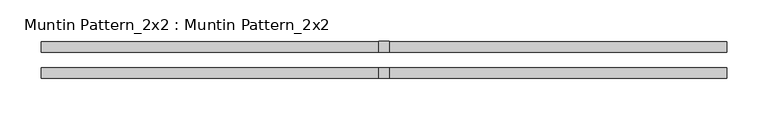
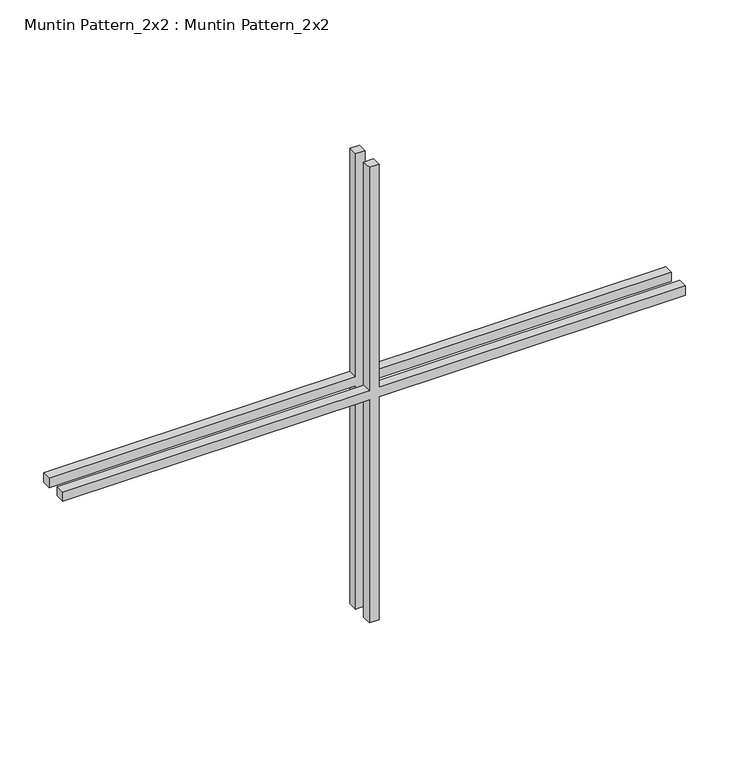
"""IFC4 building model written with IfcOpenShell, lengths in millimetres: proxy geometry, Muntin Pattern_2x2 : Muntin Pattern_2x2."""

from ifc_helpers import new_model, si_unit, frame, origin, place, context, project, spatial, polyline, outline, extrude, source, transform, mapped, element, save


def muntin_pattern_2x2_muntin_pattern_2x2_6dda0405(model_context):
    return source(origin(), model_context, "Body", "SweptSolid", [
        extrude(outline(polyline([(325.4375, -6.35), (325.4375, -412.75), (312.7375, -412.75), (312.7375, -6.35), (0.0, -6.35), (0.0, 6.35), (312.7375, 6.35), (312.7375, 412.75), (325.4375, 412.75), (325.4375, 6.35), (638.175, 6.35), (638.175, -6.35), (325.4375, -6.35)])), frame((0.0, 9.525, 0.0), z_axis=(0.0, 1.0, 0.0), x_axis=(0.0, 0.0, 1.0)), (0.0, 0.0, 1.0), 12.7),
        extrude(outline(polyline([(325.4375, -6.35), (325.4375, -412.75), (312.7375, -412.75), (312.7375, -6.35), (0.0, -6.35), (0.0, 6.35), (312.7375, 6.35), (312.7375, 412.75), (325.4375, 412.75), (325.4375, 6.35), (638.175, 6.35), (638.175, -6.35), (325.4375, -6.35)])), frame((0.0, -22.225, 0.0), z_axis=(0.0, 1.0, 0.0), x_axis=(0.0, 0.0, 1.0)), (0.0, 0.0, 1.0), 12.7),
    ])


if __name__ == "__main__":
    model = new_model("IFC4")
    model_context = context("Model", 3, world=origin())
    ifc_project = project(units=[si_unit("LENGTHUNIT", "METRE", prefix="MILLI")], contexts=[model_context])
    site = spatial("IfcSite", under=ifc_project)
    building = spatial("IfcBuilding", under=site)
    placement = place(None, origin())
    muntin_pattern_2x2_muntin_pattern_2x2_shape = muntin_pattern_2x2_muntin_pattern_2x2_6dda0405(model_context)
    element("IfcBuildingElementProxy", 1, Name="Muntin Pattern_2x2 : Muntin Pattern_2x2", ObjectType="Muntin Pattern_2x2 : Muntin Pattern_2x2", at=placement, inside=building, context=model_context, shape_type="MappedRepresentation", body=[
        mapped(muntin_pattern_2x2_muntin_pattern_2x2_shape, transform((0.0, 0.0, 0.0), x_axis=(1.0, 0.0, 0.0), y_axis=(0.0, 1.0, 0.0), z_axis=(0.0, 0.0, 1.0))),
    ])
    save(model, "model.ifc")

# Revit data of these elements
# Type "Muntin Pattern_2x2 : Muntin Pattern_2x2"
#   Width [instance default] = 4' - 0"
#   Thickness = 0' - 0 1/2"
#   Height [instance default] = 4' - 0"
#   Distance = 0' - 0 3/4"
#   Interior Material [instance default] = none
#   Exterior Material [instance default] = none
# Element 1 (IfcBuildingElementProxy, "Muntin Pattern_2x2 : Muntin Pattern_2x2")
#   Width = 2' - 8 1/2"
#   Height = 2' - 1 1/8"
#   Interior Material = Wood - Stained
#   Exterior Material = Clad - White
#   Materials on its faces: "Clad - White", "Wood - Stained"
# Materials
#   "Clad - White": class "Wood", colour RGB 242 242 238, transparency 0, Cost = 0
#   "Wood - Stained": class "Wood", colour RGB 224 178 126, transparency 0, Cost = 0
